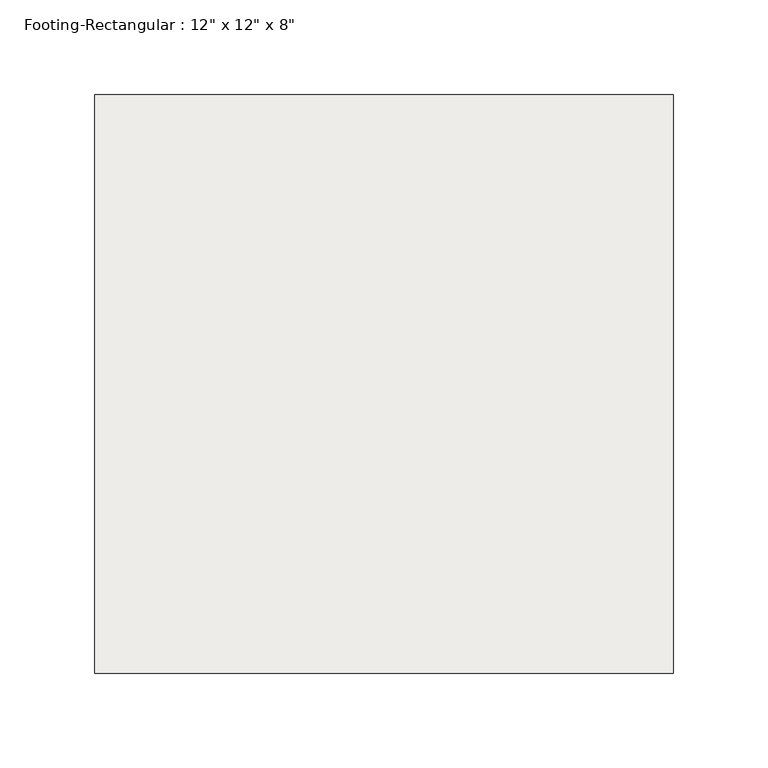
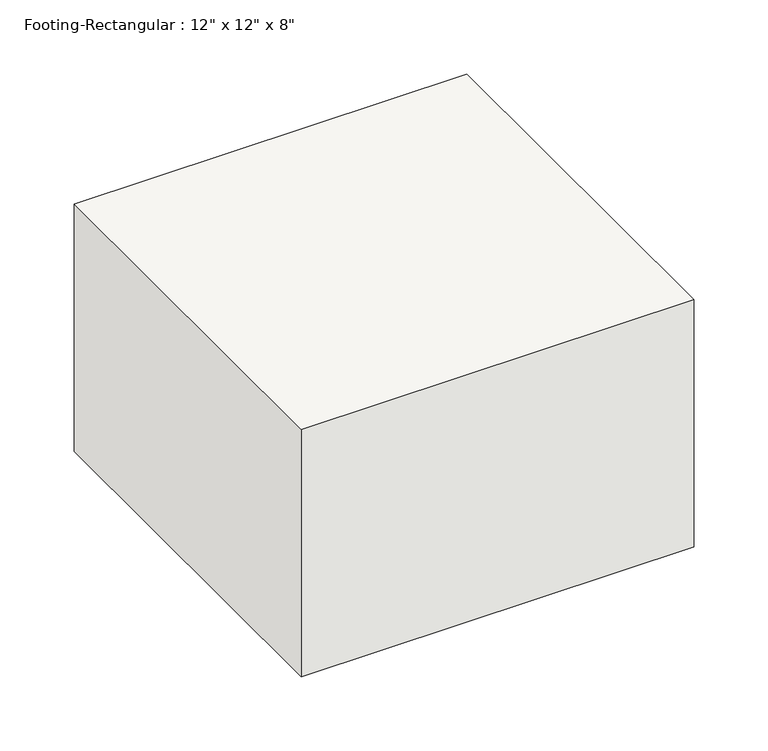
"""IFC4 building model written with IfcOpenShell, lengths in millimetres: slab geometry."""

from ifc_helpers import new_model, si_unit, frame, origin, place, context, project, spatial, polyline, outline, extrude, source, transform, mapped, element, save


def slab_3d21b0b5(model_context):
    return source(origin(), model_context, "Body", "SweptSolid", [
        extrude(outline(polyline([(152.4, 152.4), (152.4, -152.4), (-152.4, -152.4), (-152.4, 152.4), (152.4, 152.4)])), frame((0.0, 0.0, -203.2), z_axis=(0.0, 0.0, 1.0), x_axis=(1.0, 0.0, 0.0)), (0.0, 0.0, 1.0), 203.2),
    ])


if __name__ == "__main__":
    model = new_model("IFC4")
    model_context = context("Model", 3, world=origin())
    ifc_project = project(units=[si_unit("LENGTHUNIT", "METRE", prefix="MILLI")], contexts=[model_context])
    site = spatial("IfcSite", under=ifc_project)
    building = spatial("IfcBuilding", under=site)
    placement = place(None, origin())
    slab_shape = slab_3d21b0b5(model_context)
    element("IfcSlab", 1, ObjectType="Footing-Rectangular : 12\" x 12\" x 8\"", at=placement, inside=building, context=model_context, shape_type="MappedRepresentation", body=[
        mapped(slab_shape, transform((0.0, 0.0, 0.0), x_axis=(1.0, 0.0, 0.0), y_axis=(0.0, 1.0, 0.0), z_axis=(0.0, 0.0, 1.0))),
    ])
    save(model, "model.ifc")

# Revit data of these elements
# Type "Footing-Rectangular : 12\" x 12\" x 8\""
#   Assembly Code = "A1010100"
#   Width = 1' - 0"
#   Length = 1' - 0"
#   Thickness = 0' - 8"
#   Structural Material [instance default] = Concrete - Cast-in-Place Concrete
# Element 1 (IfcSlab, "Footing-Rectangular : 12\" x 12\" x 8\"")
#   Materials on its faces: "Concrete - Cast-in-Place Concrete"
# Materials
#   "Concrete - Cast-in-Place Concrete": class "Unassigned", colour RGB 192 192 192, transparency 0
